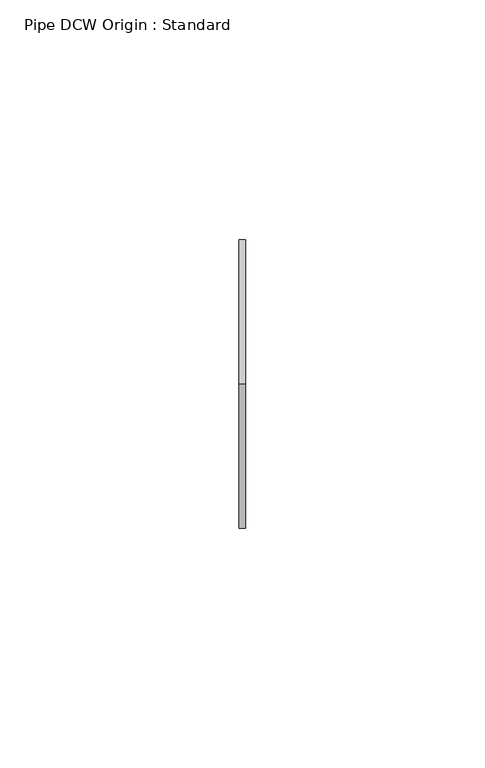
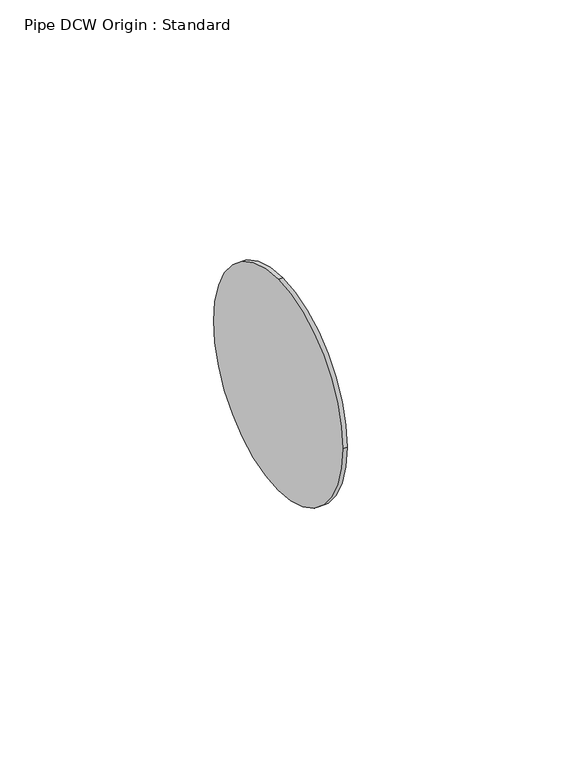
"""IFC4 building model written with IfcOpenShell, lengths in millimetres: proxy geometry, Pipe DCW Origin : Standard."""

from ifc_helpers import new_model, si_unit, point, frame, origin, origin_2d, place, context, project, spatial, circle_curve, trimmed, segment, composite_curve, outline, extrude, source, transform, mapped, element, save


def pipe_dcw_origin_standard_a8ebccfd(model_context):
    return source(origin(), model_context, "Body", "SweptSolid", [
        extrude(outline(composite_curve([segment(trimmed(circle_curve(origin_2d(), 30.1625), [point((0.0, 30.1625))], [point((30.1625, 0.0))], False, "CARTESIAN"), True, "CONTINUOUS"), segment(trimmed(circle_curve(origin_2d(), 30.1625), [point((30.1625, 0.0))], [point((0.0, -30.1625))], False, "CARTESIAN"), True, "CONTINUOUS"), segment(trimmed(circle_curve(origin_2d(), 30.1625), [point((0.0, -30.1625))], [point((-30.1625, 0.0))], False, "CARTESIAN"), True, "CONTINUOUS"), segment(trimmed(circle_curve(origin_2d(), 30.1625), [point((-30.1625, 0.0))], [point((0.0, 30.1625))], False, "CARTESIAN"), True, "CONTINUOUS")], self_intersect=False)), frame((0.0, 0.0, 0.0), z_axis=(1.0, 0.0, 0.0), x_axis=(0.0, 1.0, 0.0)), (0.0, 0.0, 1.0), 1.27),
        extrude(outline(composite_curve([segment(trimmed(circle_curve(origin_2d(), 30.1625), [point((0.0, 30.1625))], [point((30.1625, 0.0))], False, "CARTESIAN"), True, "CONTINUOUS"), segment(trimmed(circle_curve(origin_2d(), 30.1625), [point((30.1625, 0.0))], [point((0.0, -30.1625))], False, "CARTESIAN"), True, "CONTINUOUS"), segment(trimmed(circle_curve(origin_2d(), 30.1625), [point((0.0, -30.1625))], [point((-30.1625, 0.0))], False, "CARTESIAN"), True, "CONTINUOUS"), segment(trimmed(circle_curve(origin_2d(), 30.1625), [point((-30.1625, 0.0))], [point((0.0, 30.1625))], False, "CARTESIAN"), True, "CONTINUOUS")], self_intersect=False)), frame((0.0, 0.0, 0.0), z_axis=(1.0, 0.0, 0.0), x_axis=(0.0, 1.0, 0.0)), (0.0, 0.0, 1.0), 1.27),
    ])


if __name__ == "__main__":
    model = new_model("IFC4")
    model_context = context("Model", 3, world=origin())
    ifc_project = project(units=[si_unit("LENGTHUNIT", "METRE", prefix="MILLI")], contexts=[model_context])
    site = spatial("IfcSite", under=ifc_project)
    building = spatial("IfcBuilding", under=site)
    placement = place(None, origin())
    pipe_dcw_origin_standard_shape = pipe_dcw_origin_standard_a8ebccfd(model_context)
    element("IfcBuildingElementProxy", 1, Name="Pipe DCW Origin : Standard", ObjectType="Pipe DCW Origin : Standard", at=placement, inside=building, context=model_context, shape_type="MappedRepresentation", body=[
        mapped(pipe_dcw_origin_standard_shape, transform((0.0, 0.0, 0.0), x_axis=(1.0, 0.0, 0.0), y_axis=(0.0, 1.0, 0.0), z_axis=(0.0, 0.0, 1.0))),
    ])
    save(model, "model.ifc")

# Revit data of these elements
# Type "Pipe DCW Origin : Standard"
#   Lookup Table Name [instance default] = "Pipe Fitting Sizes"
#   WaterFlow [instance default] = 0 GPM
#   Radius [instance default] = 2 3/16"
#   Nominal Size [instance default] = 4"
#   Nominal Radius [instance default] = 2"
#   Insulation Thickness [instance default] = 0"
#   Insulation Radius [instance default] = 2 3/16"
#   IsCustom [instance default] = no
#   Assembly Code = ""
# Element 1 (IfcBuildingElementProxy, "Pipe DCW Origin : Standard")
#   Radius = 1 3/16"
#   Nominal Size = 2"
#   Nominal Radius = 1"
#   Insulation Radius = 1 3/16"
